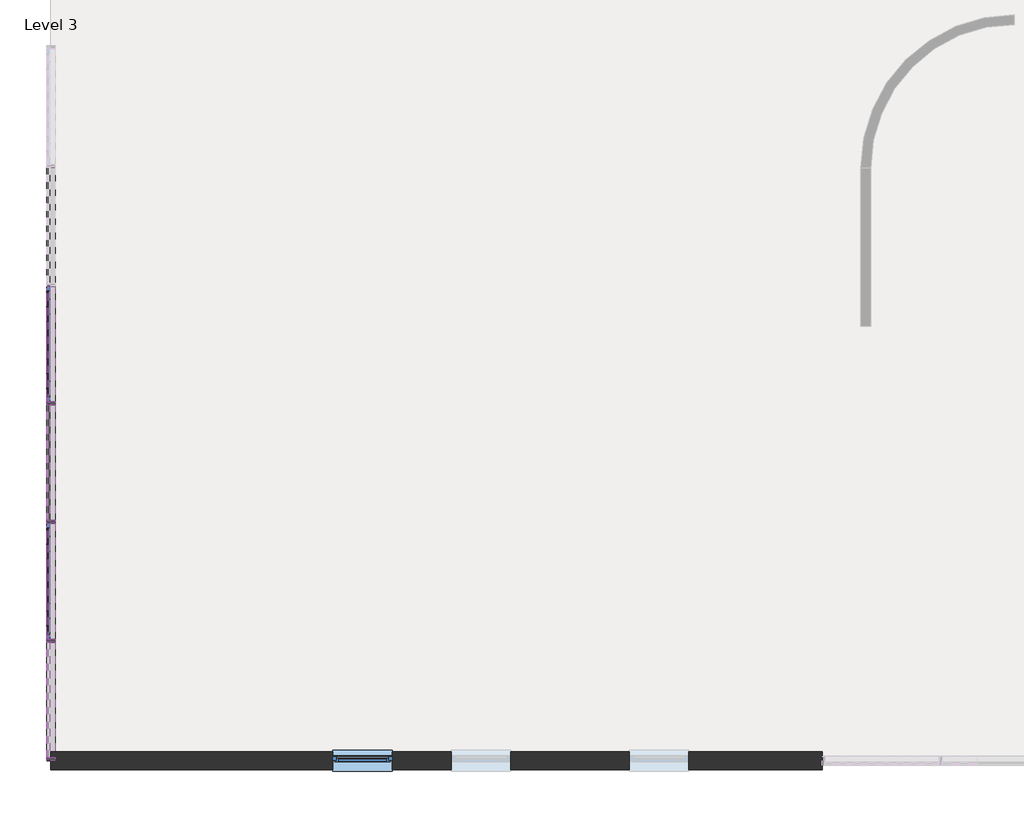
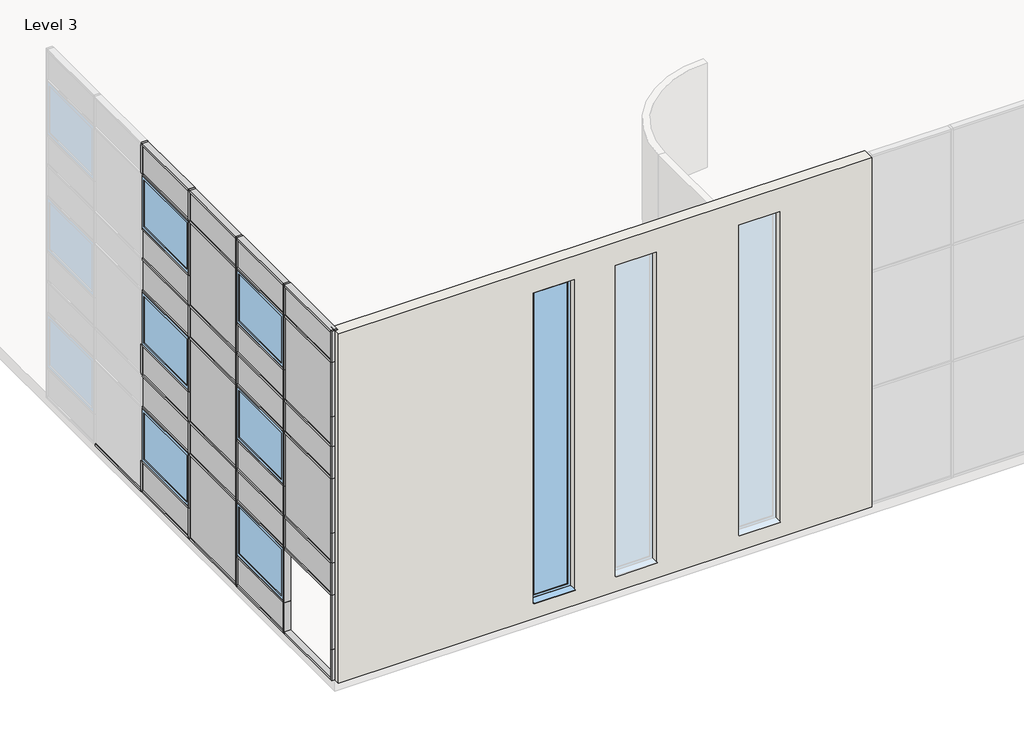
# One storey, part 1 of 5: 74 members, 23 plates, 7 windows, 1 wall.
"""IFC4 building model written with IfcOpenShell, lengths in millimetres."""

import ifcopenshell
import ifcopenshell.guid

model = None  # the IFC model being written
_history = None  # IfcOwnerHistory: only IFC2X3 demands one
_inside = {}  # id of a spatial element -> (the spatial element, [elements in it])
_under = {}  # id of a project, library or spatial element -> (it, [spatial elements below it])
_declared = {}  # id of a project -> (the project, [libraries it declares])
_typed = {}  # id of a type object -> (the type object, [elements of that type])
_made_of = {}  # id of a material, layer set ... -> (it, [elements and type objects made of it])


def new_model(schema):
    """Start an empty IFC model of exactly this schema.

    Asked for "IFC4X3", IfcOpenShell would pick the latest addendum, in which some entities
    have other attributes; the version numbers below select the first issue.
    IFC2X3 requires an IfcOwnerHistory on every rooted entity: one is made here for all.
    """
    global model, _history
    if schema == "IFC4X3":
        model = ifcopenshell.file(schema_version=(4, 3, 0, 0))
    else:
        model = ifcopenshell.file(schema=schema)
    _inside.clear()
    _under.clear()
    _declared.clear()
    _typed.clear()
    _made_of.clear()
    _history = None
    if model.schema == "IFC2X3":
        org = make("IfcOrganization", Name="unknown")
        user = make(
            "IfcPersonAndOrganization",
            ThePerson=make("IfcPerson", FamilyName="unknown"),
            TheOrganization=org,
        )
        app = make(
            "IfcApplication",
            ApplicationDeveloper=org,
            Version="unknown",
            ApplicationFullName="unknown",
            ApplicationIdentifier="unknown",
        )
        _history = make(
            "IfcOwnerHistory",
            OwningUser=user,
            OwningApplication=app,
            ChangeAction="ADDED",
            CreationDate=0,
        )
    return model


def make(cls, **values):
    """One entity of the class cls with the attributes given. An attribute that is None is left unset."""
    return model.create_entity(
        cls, **{name: value for name, value in values.items() if value is not None}
    )


def rooted(cls, **values):
    """An entity with a GlobalId (a new one), such as an element, a storey or a relation."""
    return make(cls, GlobalId=ifcopenshell.guid.new(), OwnerHistory=_history, **values)


def si_unit(unit_type, name, prefix=None):
    """IfcSIUnit, for example si_unit("LENGTHUNIT", "METRE", prefix="MILLI")."""
    return make("IfcSIUnit", UnitType=unit_type, Prefix=prefix, Name=name)


def assignment(units):
    """IfcUnitAssignment: the units of a project."""
    return None if units is None else make("IfcUnitAssignment", Units=units)


def point(xyz):
    """IfcCartesianPoint."""
    return None if xyz is None else make("IfcCartesianPoint", Coordinates=xyz)


def direction(xyz):
    """IfcDirection."""
    return None if xyz is None else make("IfcDirection", DirectionRatios=xyz)


def frame(location, z_axis=None, x_axis=None):
    """IfcAxis2Placement3D, a coordinate frame: its origin and axes. An axis left out is left unset."""
    return make(
        "IfcAxis2Placement3D",
        Location=point(location),
        Axis=direction(z_axis),
        RefDirection=direction(x_axis),
    )


def origin():
    """The frame at (0, 0, 0) with its axes left unset."""
    return frame((0.0, 0.0, 0.0))


def origin_with_axes():
    """The frame at (0, 0, 0) with the z axis (0, 0, 1) and the x axis (1, 0, 0) written out."""
    return frame((0.0, 0.0, 0.0), z_axis=(0.0, 0.0, 1.0), x_axis=(1.0, 0.0, 0.0))


def place(relative_to, where):
    """IfcLocalPlacement: puts the frame where relative to a parent placement (None: the world)."""
    return make(
        "IfcLocalPlacement", PlacementRelTo=relative_to, RelativePlacement=where
    )


def context(
    kind, dimensions, precision=None, world=None, true_north=None, identifier=None
):
    """IfcGeometricRepresentationContext, for example the 3D "Model" context."""
    return make(
        "IfcGeometricRepresentationContext",
        ContextIdentifier=identifier,
        ContextType=kind,
        CoordinateSpaceDimension=dimensions,
        Precision=precision,
        WorldCoordinateSystem=world,
        TrueNorth=true_north,
    )


def project(units=None, contexts=None):
    """IfcProject with its units and contexts."""
    return rooted(
        "IfcProject",
        Name="project",
        RepresentationContexts=contexts,
        UnitsInContext=assignment(units),
    )


def spatial(cls, under=None, at=None, **own):
    """A site, building, storey or space (cls), placed at a placement, below another one or the project."""
    s = rooted(cls, ObjectPlacement=at, **own)
    if under is not None:
        _under.setdefault(under.id(), (under, []))[1].append(s)
    return s


def polyline(points):
    """IfcPolyline through the points."""
    return make("IfcPolyline", Points=[point(p) for p in points])


def outline(outer, holes=None, kind="AREA"):
    """IfcArbitraryClosedProfileDef: a profile drawn as a closed curve; with holes, ...WithVoids."""
    if holes is None:
        return make("IfcArbitraryClosedProfileDef", ProfileType=kind, OuterCurve=outer)
    return make(
        "IfcArbitraryProfileDefWithVoids",
        ProfileType=kind,
        OuterCurve=outer,
        InnerCurves=holes,
    )


def extrude(swept, where, along, depth):
    """IfcExtrudedAreaSolid: the profile swept, set in the frame where, extruded along a direction by depth."""
    return make(
        "IfcExtrudedAreaSolid",
        SweptArea=swept,
        Position=where,
        ExtrudedDirection=direction(along),
        Depth=depth,
    )


def faces_of(points, faces, orient=None, outer=None):
    """IfcFace entities. A face is a list of loops; a loop is a list of indices into points, from 0.

    orient and outer hold one flag for each loop. By default every Orientation is true, the
    first loop of a face is its IfcFaceOuterBound and the others are IfcFaceBound.
    """
    made = []
    for i, loops in enumerate(faces):
        bounds = []
        for j, loop in enumerate(loops):
            is_outer = j == 0 if outer is None else outer[i][j]
            bounds.append(
                make(
                    "IfcFaceOuterBound" if is_outer else "IfcFaceBound",
                    Bound=make("IfcPolyLoop", Polygon=[points[k] for k in loop]),
                    Orientation=True if orient is None else orient[i][j],
                )
            )
        made.append(make("IfcFace", Bounds=bounds))
    return made


def faceted_brep(points, faces, orient=None, outer=None, voids=None):
    """IfcFacetedBrep: a solid bounded by flat faces; with voids (closed shells), ...WithVoids."""
    shared = [point(p) for p in points]
    hull = make("IfcClosedShell", CfsFaces=faces_of(shared, faces, orient, outer))
    if voids is None:
        return make("IfcFacetedBrep", Outer=hull)
    return make(
        "IfcFacetedBrepWithVoids",
        Outer=hull,
        Voids=[
            make(cls, CfsFaces=faces_of(shared, fs, o, b)) for cls, fs, o, b in voids
        ],
    )


def shape(context_of_items, identifier, shape_type, items):
    """IfcShapeRepresentation: the items that make up one representation, for example the "Body"."""
    return make(
        "IfcShapeRepresentation",
        ContextOfItems=context_of_items,
        RepresentationIdentifier=identifier,
        RepresentationType=shape_type,
        Items=items,
    )


def source(mapping_origin, context_of_items, identifier, shape_type, items):
    """IfcRepresentationMap: a shape defined once, which mapped items show again and again."""
    return make(
        "IfcRepresentationMap",
        MappingOrigin=mapping_origin,
        MappedRepresentation=shape(context_of_items, identifier, shape_type, items),
    )


def transform(
    local_origin,
    x_axis=None,
    y_axis=None,
    z_axis=None,
    scale=None,
    scale2=None,
    scale3=None,
    uniform=True,
):
    """IfcCartesianTransformationOperator3D, or its non-uniform kind. x_axis, y_axis, z_axis: its Axis1, 2, 3."""
    if uniform:
        return make(
            "IfcCartesianTransformationOperator3D",
            Axis1=direction(x_axis),
            Axis2=direction(y_axis),
            LocalOrigin=point(local_origin),
            Scale=scale,
            Axis3=direction(z_axis),
        )
    return make(
        "IfcCartesianTransformationOperator3DnonUniform",
        Axis1=direction(x_axis),
        Axis2=direction(y_axis),
        LocalOrigin=point(local_origin),
        Scale=scale,
        Axis3=direction(z_axis),
        Scale2=scale2,
        Scale3=scale3,
    )


def mapped(mapping_source, mapping_target):
    """IfcMappedItem: shows the shape of a source again, moved by a transform."""
    return make(
        "IfcMappedItem", MappingSource=mapping_source, MappingTarget=mapping_target
    )


def made_of(thing, what):
    """Note that an element or type object is made of a material, layer set ...; save() writes the relation."""
    if what is not None:
        _made_of.setdefault(what.id(), (what, []))[1].append(thing)
    return thing


def element(
    cls,
    number,
    at=None,
    inside=None,
    cuts=None,
    type_object=None,
    material=None,
    context=None,
    identifier="Body",
    shape_type=None,
    held_by="IfcProductDefinitionShape",
    body=None,
    shapes=None,
    **own,
):
    """One element of the class cls, such as IfcWall. Its Tag is "e" and its number.

    at: its placement. inside: the storey or other place that contains it. cuts: it is an
    opening in that element (IfcRelVoidsElement). A single representation is given by context,
    identifier, shape_type and body (its items); several are given by shapes. held_by: the class
    of the entity that holds the representations. save() writes the other relations.
    """
    e = rooted(cls, Tag="e%d" % number, ObjectPlacement=at, **own)
    if body is not None:
        shapes = [shape(context, identifier, shape_type, body)]
    if shapes is not None:
        e.Representation = make(held_by, Representations=shapes)
    if inside is not None:
        _inside.setdefault(inside.id(), (inside, []))[1].append(e)
    if cuts is not None:
        rooted(
            "IfcRelVoidsElement", RelatingBuildingElement=cuts, RelatedOpeningElement=e
        )
    if type_object is not None:
        _typed.setdefault(type_object.id(), (type_object, []))[1].append(e)
    return made_of(e, material)


def aggregate(whole, parts):
    """IfcRelAggregates: a whole, such as a stair, and the parts it consists of."""
    return rooted("IfcRelAggregates", RelatingObject=whole, RelatedObjects=parts)


def save(model, path):
    """Write the relations noted so far, then the file.

    IfcRelAggregates (storeys below a building ...), IfcRelContainedInSpatialStructure (elements
    in a storey), IfcRelDefinesByType, IfcRelAssociatesMaterial and IfcRelDeclares: one each for
    every whole, place, type object, material and project.
    """
    for whole, parts in _under.values():
        aggregate(whole, parts)
    for where, things in _inside.values():
        rooted(
            "IfcRelContainedInSpatialStructure",
            RelatedElements=things,
            RelatingStructure=where,
        )
    for kind, things in _typed.values():
        rooted("IfcRelDefinesByType", RelatedObjects=things, RelatingType=kind)
    for what, things in _made_of.values():
        rooted("IfcRelAssociatesMaterial", RelatedObjects=things, RelatingMaterial=what)
    for by, libraries in _declared.values():
        rooted("IfcRelDeclares", RelatingContext=by, RelatedDefinitions=libraries)
    model.write(path)


def rectangular_mullion_50_x_150mm_0967fd3c(model_context):
    return source(origin(), model_context, "Body", "SweptSolid", [
        extrude(outline(polyline([(0.0, 75.0), (0.0, -75.0), (-50.0, -75.0), (-50.0, 75.0), (0.0, 75.0)])), frame((0.0, 0.0, -1950.0000003), z_axis=(0.0, 0.0, 1.0), x_axis=(1.0, 0.0, 0.0)), (0.0, 0.0, 1.0), 1950.0000003),
    ])


def rectangular_mullion_50_x_150mm_f1645b81(model_context):
    return source(origin(), model_context, "Body", "SweptSolid", [
        extrude(outline(polyline([(25.0, 75.0), (25.0, -75.0), (-25.0, -75.0), (-25.0, 75.0), (25.0, 75.0)])), frame((0.0, 0.0, -1950.0000003), z_axis=(0.0, 0.0, 1.0), x_axis=(1.0, 0.0, 0.0)), (0.0, 0.0, 1.0), 1950.0000003),
    ])


def rectangular_mullion_50_x_150mm_14f10ac7(model_context):
    return source(origin(), model_context, "Body", "SweptSolid", [
        extrude(outline(polyline([(25.0, 75.0), (25.0, -75.0), (-25.0, -75.0), (-25.0, 75.0), (25.0, 75.0)])), frame((0.0, 0.0, -800.0), z_axis=(0.0, 0.0, 1.0), x_axis=(1.0, 0.0, 0.0)), (0.0, 0.0, 1.0), 800.0),
    ])


def rectangular_mullion_50_x_150mm_6270d9f9(model_context):
    return source(origin(), model_context, "Body", "SweptSolid", [
        extrude(outline(polyline([(25.0, 75.0), (25.0, -75.0), (-25.0, -75.0), (-25.0, 75.0), (25.0, 75.0)])), frame((0.0, 0.0, -775.0), z_axis=(0.0, 0.0, 1.0), x_axis=(1.0, 0.0, 0.0)), (0.0, 0.0, 1.0), 775.0),
    ])


def rectangular_mullion_50_x_150mm_80d7b263(model_context):
    return source(origin(), model_context, "Body", "SweptSolid", [
        extrude(outline(polyline([(25.0, 75.0), (25.0, -75.0), (-25.0, -75.0), (-25.0, 75.0), (25.0, 75.0)])), frame((0.0, 0.0, -1400.0), z_axis=(0.0, 0.0, 1.0), x_axis=(1.0, 0.0, 0.0)), (0.0, 0.0, 1.0), 1400.0),
    ])


def rectangular_mullion_50_x_150mm_9c26cac3(model_context):
    return source(origin(), model_context, "Body", "SweptSolid", [
        extrude(outline(polyline([(25.0, 75.0), (25.0, -75.0), (-25.0, -75.0), (-25.0, 75.0), (25.0, 75.0)])), frame((0.0, 0.0, -825.0), z_axis=(0.0, 0.0, 1.0), x_axis=(1.0, 0.0, 0.0)), (0.0, 0.0, 1.0), 825.0),
    ])


def rectangular_mullion_50_x_150mm_6ffebc0f(model_context):
    return source(origin(), model_context, "Body", "SweptSolid", [
        extrude(outline(polyline([(0.0, 75.0), (0.0, -75.0), (-50.0, -75.0), (-50.0, 75.0), (0.0, 75.0)])), frame((0.0, 0.0, -800.0), z_axis=(0.0, 0.0, 1.0), x_axis=(1.0, 0.0, 0.0)), (0.0, 0.0, 1.0), 800.0),
    ])


def rectangular_mullion_50_x_150mm_0ac3c94c(model_context):
    return source(origin(), model_context, "Body", "SweptSolid", [
        extrude(outline(polyline([(0.0, 75.0), (0.0, -75.0), (-50.0, -75.0), (-50.0, 75.0), (0.0, 75.0)])), frame((0.0, 0.0, -1400.0), z_axis=(0.0, 0.0, 1.0), x_axis=(1.0, 0.0, 0.0)), (0.0, 0.0, 1.0), 1400.0),
    ])


def rectangular_mullion_50_x_150mm_4883e7f1(model_context):
    return source(origin(), model_context, "Body", "SweptSolid", [
        extrude(outline(polyline([(0.0, 75.0), (0.0, -75.0), (-50.0, -75.0), (-50.0, 75.0), (0.0, 75.0)])), frame((0.0, 0.0, -825.0), z_axis=(0.0, 0.0, 1.0), x_axis=(1.0, 0.0, 0.0)), (0.0, 0.0, 1.0), 825.0),
    ])


def rectangular_mullion_50_x_150mm_5dc04e1f(model_context):
    return source(origin(), model_context, "Body", "SweptSolid", [
        extrude(outline(polyline([(0.0, 75.0), (0.0, -75.0), (-50.0, -75.0), (-50.0, 75.0), (0.0, 75.0)])), frame((0.0, 0.0, -775.0), z_axis=(0.0, 0.0, 1.0), x_axis=(1.0, 0.0, 0.0)), (0.0, 0.0, 1.0), 775.0),
    ])


def system_panel_glazed_1e38db9b(model_context):
    return source(origin(), model_context, "Body", "SweptSolid", [
        extrude(outline(polyline([(0.0, -975.0000002), (0.0, 975.0000002), (750.0, 975.0000002), (2125.0, 975.0000002), (2125.0, -975.0000002), (750.0, -975.0000002), (0.0, -975.0000002)])), frame((0.0, 24.5, 0.0), z_axis=(0.0, 1.0, 0.0), x_axis=(0.0, 0.0, 1.0)), (0.0, 0.0, 1.0), 25.0),
    ])


def system_panel_glazed_bc1ebc0c(model_context):
    return source(origin(), model_context, "Body", "SweptSolid", [
        extrude(outline(polyline([(975.0000002, 24.5), (-975.0000002, 24.5), (-975.0000002, 49.5), (975.0000002, 49.5), (975.0000002, 24.5)])), origin_with_axes(), (0.0, 0.0, 1.0), 725.0),
    ])


def system_panel_glazed_d82c9dbb(model_context):
    return source(origin(), model_context, "Body", "SweptSolid", [
        extrude(outline(polyline([(975.0000002, 24.5), (-975.0000002, 24.5), (-975.0000002, 49.5), (975.0000002, 49.5), (975.0000002, 24.5)])), origin_with_axes(), (0.0, 0.0, 1.0), 775.0),
    ])


def m_curtain_wall_awning_m_curtain_wall_awning_db665c81(model_context):
    return source(origin(), model_context, "Body", "SweptSolid", [
        extrude(outline(polyline([(900.0, 44.05), (-900.0, 44.05), (-900.0, 56.75), (900.0, 56.75), (900.0, 44.05)])), frame((0.0, 0.0, 75.0), z_axis=(0.0, 0.0, 1.0), x_axis=(1.0, 0.0, 0.0)), (0.0, 0.0, 1.0), 1200.0),
        extrude(outline(polyline([(1350.0, -975.0), (0.0, -975.0), (0.0, 975.0), (1350.0, 975.0), (1350.0, -975.0)]), holes=[polyline([(1275.0, -900.0), (1275.0, 900.0), (75.0, 900.0), (75.0, -900.0), (1275.0, -900.0)])]), frame((0.0, 25.0, 0.0), z_axis=(0.0, 1.0, 0.0), x_axis=(0.0, 0.0, 1.0)), (0.0, 0.0, 1.0), 50.0),
    ])


def window_variable_standard_9eb8f332(model_context):
    return source(origin(), model_context, "Body", "SolidModel", [
        extrude(outline(polyline([(9000.0, 500.0), (9000.0, -500.0), (1000.0, -500.0), (1000.0, 500.0), (9000.0, 500.0)]), holes=[polyline([(8920.0, 440.0), (1080.0, 440.0), (1080.0, -440.0), (8920.0, -440.0), (8920.0, 440.0)])]), frame((0.0, -70.0, 0.0), z_axis=(0.0, 1.0, 0.0), x_axis=(0.0, 0.0, 1.0)), (0.0, 0.0, 1.0), 60.0),
        faceted_brep([(470.0, -10.0, 8950.0), (470.0, -10.0, 1050.0), (470.0, 20.0, 1050.0), (470.0, 20.0, 8950.0), (-470.0, 20.0, 1050.0), (-470.0, 20.0, 8950.0), (410.0, 20.0, 1110.0), (410.0, 20.0, 8890.0), (-410.0, 20.0, 8890.0), (-410.0, 20.0, 1110.0), (-470.0, -10.0, 1050.0), (-470.0, -10.0, 8950.0), (440.0, -10.0, 8920.0), (440.0, -10.0, 1080.0), (-440.0, -10.0, 1080.0), (-440.0, -10.0, 8920.0), (440.0, -40.0, 8920.0), (440.0, -40.0, 1080.0), (-440.0, -40.0, 1080.0), (-440.0, -40.0, 8920.0), (410.0, -40.0, 8890.0), (410.0, -40.0, 1110.0), (-410.0, -40.0, 1110.0), (-410.0, -40.0, 8890.0)], [[[0, 1, 2, 3]], [[3, 2, 4, 5], [6, 7, 8, 9]], [[1, 10, 4, 2]], [[1, 0, 11, 10], [12, 13, 14, 15]], [[16, 17, 13, 12]], [[17, 18, 14, 13]], [[17, 16, 19, 18], [20, 21, 22, 23]], [[7, 6, 21, 20]], [[6, 9, 22, 21]], [[10, 11, 5, 4]], [[18, 19, 15, 14]], [[9, 8, 23, 22]], [[11, 0, 3, 5]], [[19, 16, 12, 15]], [[8, 7, 20, 23]]]),
        extrude(outline(polyline([(-500.0, 180.0), (500.0, 180.0), (500.0, -10.0), (-500.0, -10.0), (-500.0, 180.0)])), frame((0.0, 0.0, 1005.0), z_axis=(0.0, 0.0, 1.0), x_axis=(1.0, 0.0, 0.0)), (0.0, 0.0, 1.0), 15.0),
        extrude(outline(polyline([(-80.0221543, 1020.0), (-70.0, 1020.0), (-70.0, 1018.0), (-79.8240723, 1018.0), (-178.0, 998.3604634), (-178.0, 990.0), (-180.0, 990.0), (-180.0, 1000.0), (-80.0221543, 1020.0)])), frame((-500.0, 0.0, 0.0), z_axis=(1.0, 0.0, 0.0), x_axis=(0.0, 1.0, 0.0)), (0.0, 0.0, 1.0), 1000.0),
        extrude(outline(polyline([(410.0, 5.0), (410.0, -25.0), (-410.0, -25.0), (-410.0, 5.0), (410.0, 5.0)])), frame((0.0, 0.0, 1110.0), z_axis=(0.0, 0.0, 1.0), x_axis=(1.0, 0.0, 0.0)), (0.0, 0.0, 1.0), 7780.0),
    ])


model = new_model("IFC4")

# Units and contexts
model_context = context("Model", 3, world=origin())
ifc_project = project(units=[si_unit("LENGTHUNIT", "METRE", prefix="MILLI")], contexts=[model_context])

# Site, building, storey
site = spatial("IfcSite", under=ifc_project)
building = spatial("IfcBuilding", under=site)
storey = spatial("IfcBuildingStorey", under=building, Name="Level 3", Elevation=6000.0)

# Members
placement = place(None, origin())
rectangular_mullion_50_x_150mm_shape = rectangular_mullion_50_x_150mm_0967fd3c(model_context)
element("IfcMember", 1, ObjectType="Rectangular Mullion : 50 x 150mm", at=placement, inside=storey, context=model_context, shape_type="MappedRepresentation", body=[
    mapped(rectangular_mullion_50_x_150mm_shape, transform((-6732.0028633, -9951.242277, 6000.0), x_axis=(0.0, 0.0, -1.0), y_axis=(1.0, 0.0, 0.0), z_axis=(0.0, -1.0, 0.0))),
])
element("IfcMember", 2, ObjectType="Rectangular Mullion : 50 x 150mm", at=placement, inside=storey, context=model_context, shape_type="MappedRepresentation", body=[
    mapped(rectangular_mullion_50_x_150mm_shape, transform((-6732.0028633, -7951.2422767, 6000.0), x_axis=(0.0, 0.0, -1.0), y_axis=(1.0, 0.0, 0.0), z_axis=(0.0, -1.0, 0.0))),
])
element("IfcMember", 3, ObjectType="Rectangular Mullion : 50 x 150mm", at=placement, inside=storey, context=model_context, shape_type="MappedRepresentation", body=[
    mapped(rectangular_mullion_50_x_150mm_shape, transform((-6732.0028633, -5951.2422767, 6000.0), x_axis=(0.0, 0.0, -1.0), y_axis=(1.0, 0.0, 0.0), z_axis=(0.0, -1.0, 0.0))),
])
element("IfcMember", 4, ObjectType="Rectangular Mullion : 50 x 150mm", at=placement, inside=storey, context=model_context, shape_type="MappedRepresentation", body=[
    mapped(rectangular_mullion_50_x_150mm_shape, transform((-6732.0028633, -3951.2422767, 6000.0), x_axis=(0.0, 0.0, -1.0), y_axis=(1.0, 0.0, 0.0), z_axis=(0.0, -1.0, 0.0))),
])
element("IfcMember", 5, ObjectType="Rectangular Mullion : 50 x 150mm", at=placement, inside=storey, context=model_context, shape_type="MappedRepresentation", body=[
    mapped(rectangular_mullion_50_x_150mm_shape, transform((-6732.0028633, -1951.2422767, 6000.0), x_axis=(0.0, 0.0, -1.0), y_axis=(1.0, 0.0, 0.0), z_axis=(0.0, -1.0, 0.0))),
])
rectangular_mullion_50_x_150mm_2_shape = rectangular_mullion_50_x_150mm_f1645b81(model_context)
element("IfcMember", 6, ObjectType="Rectangular Mullion : 50 x 150mm", at=placement, inside=storey, context=model_context, shape_type="MappedRepresentation", body=[
    mapped(rectangular_mullion_50_x_150mm_2_shape, transform((-6732.0028633, -8001.2422767, 14200.0), x_axis=(0.0, 0.0, 1.0), y_axis=(1.0, 0.0, 0.0), z_axis=(0.0, 1.0, 0.0))),
])
element("IfcMember", 7, ObjectType="Rectangular Mullion : 50 x 150mm", at=placement, inside=storey, context=model_context, shape_type="MappedRepresentation", body=[
    mapped(rectangular_mullion_50_x_150mm_2_shape, transform((-6732.0028633, -6001.2422767, 14200.0), x_axis=(0.0, 0.0, 1.0), y_axis=(1.0, 0.0, 0.0), z_axis=(0.0, 1.0, 0.0))),
])
element("IfcMember", 8, ObjectType="Rectangular Mullion : 50 x 150mm", at=placement, inside=storey, context=model_context, shape_type="MappedRepresentation", body=[
    mapped(rectangular_mullion_50_x_150mm_2_shape, transform((-6732.0028633, -4001.2422767, 14200.0), x_axis=(0.0, 0.0, 1.0), y_axis=(1.0, 0.0, 0.0), z_axis=(0.0, 1.0, 0.0))),
])
element("IfcMember", 9, ObjectType="Rectangular Mullion : 50 x 150mm", at=placement, inside=storey, context=model_context, shape_type="MappedRepresentation", body=[
    mapped(rectangular_mullion_50_x_150mm_2_shape, transform((-6732.0028633, -2001.2422767, 14200.0), x_axis=(0.0, 0.0, 1.0), y_axis=(1.0, 0.0, 0.0), z_axis=(0.0, 1.0, 0.0))),
])
element("IfcMember", 10, ObjectType="Rectangular Mullion : 50 x 150mm", at=placement, inside=storey, context=model_context, shape_type="MappedRepresentation", body=[
    mapped(rectangular_mullion_50_x_150mm_2_shape, transform((-6732.0028633, -8001.2422767, 9025.0), x_axis=(0.0, 0.0, 1.0), y_axis=(1.0, 0.0, 0.0), z_axis=(0.0, 1.0, 0.0))),
])
element("IfcMember", 11, ObjectType="Rectangular Mullion : 50 x 150mm", at=placement, inside=storey, context=model_context, shape_type="MappedRepresentation", body=[
    mapped(rectangular_mullion_50_x_150mm_2_shape, transform((-6732.0028633, -6001.2422767, 9025.0), x_axis=(0.0, 0.0, 1.0), y_axis=(1.0, 0.0, 0.0), z_axis=(0.0, 1.0, 0.0))),
])
element("IfcMember", 12, ObjectType="Rectangular Mullion : 50 x 150mm", at=placement, inside=storey, context=model_context, shape_type="MappedRepresentation", body=[
    mapped(rectangular_mullion_50_x_150mm_2_shape, transform((-6732.0028633, -4001.2422767, 9025.0), x_axis=(0.0, 0.0, 1.0), y_axis=(1.0, 0.0, 0.0), z_axis=(0.0, 1.0, 0.0))),
])
element("IfcMember", 13, ObjectType="Rectangular Mullion : 50 x 150mm", at=placement, inside=storey, context=model_context, shape_type="MappedRepresentation", body=[
    mapped(rectangular_mullion_50_x_150mm_2_shape, transform((-6732.0028633, -2001.2422767, 9025.0), x_axis=(0.0, 0.0, 1.0), y_axis=(1.0, 0.0, 0.0), z_axis=(0.0, 1.0, 0.0))),
])
element("IfcMember", 14, ObjectType="Rectangular Mullion : 50 x 150mm", at=placement, inside=storey, context=model_context, shape_type="MappedRepresentation", body=[
    mapped(rectangular_mullion_50_x_150mm_2_shape, transform((-6732.0028633, -8001.2422767, 12025.0), x_axis=(0.0, 0.0, 1.0), y_axis=(1.0, 0.0, 0.0), z_axis=(0.0, 1.0, 0.0))),
])
element("IfcMember", 15, ObjectType="Rectangular Mullion : 50 x 150mm", at=placement, inside=storey, context=model_context, shape_type="MappedRepresentation", body=[
    mapped(rectangular_mullion_50_x_150mm_2_shape, transform((-6732.0028633, -6001.2422767, 12025.0), x_axis=(0.0, 0.0, 1.0), y_axis=(1.0, 0.0, 0.0), z_axis=(0.0, 1.0, 0.0))),
])
element("IfcMember", 16, ObjectType="Rectangular Mullion : 50 x 150mm", at=placement, inside=storey, context=model_context, shape_type="MappedRepresentation", body=[
    mapped(rectangular_mullion_50_x_150mm_2_shape, transform((-6732.0028633, -4001.2422767, 12025.0), x_axis=(0.0, 0.0, 1.0), y_axis=(1.0, 0.0, 0.0), z_axis=(0.0, 1.0, 0.0))),
])
element("IfcMember", 17, ObjectType="Rectangular Mullion : 50 x 150mm", at=placement, inside=storey, context=model_context, shape_type="MappedRepresentation", body=[
    mapped(rectangular_mullion_50_x_150mm_2_shape, transform((-6732.0028633, -2001.2422767, 12025.0), x_axis=(0.0, 0.0, 1.0), y_axis=(1.0, 0.0, 0.0), z_axis=(0.0, 1.0, 0.0))),
])
element("IfcMember", 18, ObjectType="Rectangular Mullion : 50 x 150mm", at=placement, inside=storey, context=model_context, shape_type="MappedRepresentation", body=[
    mapped(rectangular_mullion_50_x_150mm_2_shape, transform((-6732.0028633, -6001.2422767, 12800.0), x_axis=(0.0, 0.0, 1.0), y_axis=(1.0, 0.0, 0.0), z_axis=(0.0, 1.0, 0.0))),
])
element("IfcMember", 19, ObjectType="Rectangular Mullion : 50 x 150mm", at=placement, inside=storey, context=model_context, shape_type="MappedRepresentation", body=[
    mapped(rectangular_mullion_50_x_150mm_2_shape, transform((-6732.0028633, -2001.2422767, 12800.0), x_axis=(0.0, 0.0, 1.0), y_axis=(1.0, 0.0, 0.0), z_axis=(0.0, 1.0, 0.0))),
])
element("IfcMember", 20, ObjectType="Rectangular Mullion : 50 x 150mm", at=placement, inside=storey, context=model_context, shape_type="MappedRepresentation", body=[
    mapped(rectangular_mullion_50_x_150mm_2_shape, transform((-6732.0028633, -8001.2422767, 11200.0), x_axis=(0.0, 0.0, 1.0), y_axis=(1.0, 0.0, 0.0), z_axis=(0.0, 1.0, 0.0))),
])
element("IfcMember", 21, ObjectType="Rectangular Mullion : 50 x 150mm", at=placement, inside=storey, context=model_context, shape_type="MappedRepresentation", body=[
    mapped(rectangular_mullion_50_x_150mm_2_shape, transform((-6732.0028633, -6001.2422767, 11200.0), x_axis=(0.0, 0.0, 1.0), y_axis=(1.0, 0.0, 0.0), z_axis=(0.0, 1.0, 0.0))),
])
element("IfcMember", 22, ObjectType="Rectangular Mullion : 50 x 150mm", at=placement, inside=storey, context=model_context, shape_type="MappedRepresentation", body=[
    mapped(rectangular_mullion_50_x_150mm_2_shape, transform((-6732.0028633, -4001.2422767, 11200.0), x_axis=(0.0, 0.0, 1.0), y_axis=(1.0, 0.0, 0.0), z_axis=(0.0, 1.0, 0.0))),
])
element("IfcMember", 23, ObjectType="Rectangular Mullion : 50 x 150mm", at=placement, inside=storey, context=model_context, shape_type="MappedRepresentation", body=[
    mapped(rectangular_mullion_50_x_150mm_2_shape, transform((-6732.0028633, -2001.2422767, 11200.0), x_axis=(0.0, 0.0, 1.0), y_axis=(1.0, 0.0, 0.0), z_axis=(0.0, 1.0, 0.0))),
])
element("IfcMember", 24, ObjectType="Rectangular Mullion : 50 x 150mm", at=placement, inside=storey, context=model_context, shape_type="MappedRepresentation", body=[
    mapped(rectangular_mullion_50_x_150mm_2_shape, transform((-6732.0028633, -6001.2422767, 9800.0), x_axis=(0.0, 0.0, 1.0), y_axis=(1.0, 0.0, 0.0), z_axis=(0.0, 1.0, 0.0))),
])
element("IfcMember", 25, ObjectType="Rectangular Mullion : 50 x 150mm", at=placement, inside=storey, context=model_context, shape_type="MappedRepresentation", body=[
    mapped(rectangular_mullion_50_x_150mm_2_shape, transform((-6732.0028633, -2001.2422767, 9800.0), x_axis=(0.0, 0.0, 1.0), y_axis=(1.0, 0.0, 0.0), z_axis=(0.0, 1.0, 0.0))),
])
element("IfcMember", 26, ObjectType="Rectangular Mullion : 50 x 150mm", at=placement, inside=storey, context=model_context, shape_type="MappedRepresentation", body=[
    mapped(rectangular_mullion_50_x_150mm_2_shape, transform((-6732.0028633, -8001.2422767, 8200.0), x_axis=(0.0, 0.0, 1.0), y_axis=(1.0, 0.0, 0.0), z_axis=(0.0, 1.0, 0.0))),
])
element("IfcMember", 27, ObjectType="Rectangular Mullion : 50 x 150mm", at=placement, inside=storey, context=model_context, shape_type="MappedRepresentation", body=[
    mapped(rectangular_mullion_50_x_150mm_2_shape, transform((-6732.0028633, -6001.2422767, 8200.0), x_axis=(0.0, 0.0, 1.0), y_axis=(1.0, 0.0, 0.0), z_axis=(0.0, 1.0, 0.0))),
])
element("IfcMember", 28, ObjectType="Rectangular Mullion : 50 x 150mm", at=placement, inside=storey, context=model_context, shape_type="MappedRepresentation", body=[
    mapped(rectangular_mullion_50_x_150mm_2_shape, transform((-6732.0028633, -4001.2422767, 8200.0), x_axis=(0.0, 0.0, 1.0), y_axis=(1.0, 0.0, 0.0), z_axis=(0.0, 1.0, 0.0))),
])
element("IfcMember", 29, ObjectType="Rectangular Mullion : 50 x 150mm", at=placement, inside=storey, context=model_context, shape_type="MappedRepresentation", body=[
    mapped(rectangular_mullion_50_x_150mm_2_shape, transform((-6732.0028633, -2001.2422767, 8200.0), x_axis=(0.0, 0.0, 1.0), y_axis=(1.0, 0.0, 0.0), z_axis=(0.0, 1.0, 0.0))),
])
element("IfcMember", 30, ObjectType="Rectangular Mullion : 50 x 150mm", at=placement, inside=storey, context=model_context, shape_type="MappedRepresentation", body=[
    mapped(rectangular_mullion_50_x_150mm_2_shape, transform((-6732.0028633, -6001.2422767, 6800.0), x_axis=(0.0, 0.0, 1.0), y_axis=(1.0, 0.0, 0.0), z_axis=(0.0, 1.0, 0.0))),
])
element("IfcMember", 31, ObjectType="Rectangular Mullion : 50 x 150mm", at=placement, inside=storey, context=model_context, shape_type="MappedRepresentation", body=[
    mapped(rectangular_mullion_50_x_150mm_2_shape, transform((-6732.0028633, -2001.2422767, 6800.0), x_axis=(0.0, 0.0, 1.0), y_axis=(1.0, 0.0, 0.0), z_axis=(0.0, 1.0, 0.0))),
])
rectangular_mullion_50_x_150mm_3_shape = rectangular_mullion_50_x_150mm_14f10ac7(model_context)
element("IfcMember", 32, ObjectType="Rectangular Mullion : 50 x 150mm", at=placement, inside=storey, context=model_context, shape_type="MappedRepresentation", body=[
    mapped(rectangular_mullion_50_x_150mm_3_shape, transform((-6732.0028633, -7976.2422767, 6000.0), x_axis=(0.0, 1.0, 0.0), y_axis=(1.0, 0.0, 0.0), z_axis=(0.0, 0.0, -1.0))),
])
element("IfcMember", 33, ObjectType="Rectangular Mullion : 50 x 150mm", at=placement, inside=storey, context=model_context, shape_type="MappedRepresentation", body=[
    mapped(rectangular_mullion_50_x_150mm_3_shape, transform((-6732.0028633, -5976.2422767, 6000.0), x_axis=(0.0, 1.0, 0.0), y_axis=(1.0, 0.0, 0.0), z_axis=(0.0, 0.0, -1.0))),
])
element("IfcMember", 34, ObjectType="Rectangular Mullion : 50 x 150mm", at=placement, inside=storey, context=model_context, shape_type="MappedRepresentation", body=[
    mapped(rectangular_mullion_50_x_150mm_3_shape, transform((-6732.0028633, -3976.2422767, 6000.0), x_axis=(0.0, 1.0, 0.0), y_axis=(1.0, 0.0, 0.0), z_axis=(0.0, 0.0, -1.0))),
])
element("IfcMember", 35, ObjectType="Rectangular Mullion : 50 x 150mm", at=placement, inside=storey, context=model_context, shape_type="MappedRepresentation", body=[
    mapped(rectangular_mullion_50_x_150mm_3_shape, transform((-6732.0028633, -1976.2422767, 6000.0), x_axis=(0.0, 1.0, 0.0), y_axis=(1.0, 0.0, 0.0), z_axis=(0.0, 0.0, -1.0))),
])
element("IfcMember", 36, ObjectType="Rectangular Mullion : 50 x 150mm", at=placement, inside=storey, context=model_context, shape_type="MappedRepresentation", body=[
    mapped(rectangular_mullion_50_x_150mm_shape, transform((-6732.0028633, -8001.2422767, 15000.0), x_axis=(0.0, 0.0, 1.0), y_axis=(1.0, 0.0, 0.0), z_axis=(0.0, 1.0, 0.0))),
])
element("IfcMember", 37, ObjectType="Rectangular Mullion : 50 x 150mm", at=placement, inside=storey, context=model_context, shape_type="MappedRepresentation", body=[
    mapped(rectangular_mullion_50_x_150mm_shape, transform((-6732.0028633, -6001.2422767, 15000.0), x_axis=(0.0, 0.0, 1.0), y_axis=(1.0, 0.0, 0.0), z_axis=(0.0, 1.0, 0.0))),
])
element("IfcMember", 38, ObjectType="Rectangular Mullion : 50 x 150mm", at=placement, inside=storey, context=model_context, shape_type="MappedRepresentation", body=[
    mapped(rectangular_mullion_50_x_150mm_shape, transform((-6732.0028633, -4001.2422767, 15000.0), x_axis=(0.0, 0.0, 1.0), y_axis=(1.0, 0.0, 0.0), z_axis=(0.0, 1.0, 0.0))),
])
element("IfcMember", 39, ObjectType="Rectangular Mullion : 50 x 150mm", at=placement, inside=storey, context=model_context, shape_type="MappedRepresentation", body=[
    mapped(rectangular_mullion_50_x_150mm_shape, transform((-6732.0028633, -2001.2422767, 15000.0), x_axis=(0.0, 0.0, 1.0), y_axis=(1.0, 0.0, 0.0), z_axis=(0.0, 1.0, 0.0))),
])
element("IfcMember", 40, ObjectType="Rectangular Mullion : 50 x 150mm", at=placement, inside=storey, context=model_context, shape_type="MappedRepresentation", body=[
    mapped(rectangular_mullion_50_x_150mm_3_shape, transform((-6732.0028633, -7976.2422767, 14200.0), x_axis=(0.0, 1.0, 0.0), y_axis=(1.0, 0.0, 0.0), z_axis=(0.0, 0.0, -1.0))),
])
element("IfcMember", 41, ObjectType="Rectangular Mullion : 50 x 150mm", at=placement, inside=storey, context=model_context, shape_type="MappedRepresentation", body=[
    mapped(rectangular_mullion_50_x_150mm_3_shape, transform((-6732.0028633, -5976.2422767, 14200.0), x_axis=(0.0, 1.0, 0.0), y_axis=(1.0, 0.0, 0.0), z_axis=(0.0, 0.0, -1.0))),
])
element("IfcMember", 42, ObjectType="Rectangular Mullion : 50 x 150mm", at=placement, inside=storey, context=model_context, shape_type="MappedRepresentation", body=[
    mapped(rectangular_mullion_50_x_150mm_3_shape, transform((-6732.0028633, -3976.2422767, 14200.0), x_axis=(0.0, 1.0, 0.0), y_axis=(1.0, 0.0, 0.0), z_axis=(0.0, 0.0, -1.0))),
])
element("IfcMember", 43, ObjectType="Rectangular Mullion : 50 x 150mm", at=placement, inside=storey, context=model_context, shape_type="MappedRepresentation", body=[
    mapped(rectangular_mullion_50_x_150mm_3_shape, transform((-6732.0028633, -1976.2422767, 14200.0), x_axis=(0.0, 1.0, 0.0), y_axis=(1.0, 0.0, 0.0), z_axis=(0.0, 0.0, -1.0))),
])
rectangular_mullion_50_x_150mm_4_shape = rectangular_mullion_50_x_150mm_6270d9f9(model_context)
element("IfcMember", 44, ObjectType="Rectangular Mullion : 50 x 150mm", at=placement, inside=storey, context=model_context, shape_type="MappedRepresentation", body=[
    mapped(rectangular_mullion_50_x_150mm_4_shape, transform((-6732.0028633, -7976.2422767, 9025.0), x_axis=(0.0, 1.0, 0.0), y_axis=(1.0, 0.0, 0.0), z_axis=(0.0, 0.0, -1.0))),
])
element("IfcMember", 45, ObjectType="Rectangular Mullion : 50 x 150mm", at=placement, inside=storey, context=model_context, shape_type="MappedRepresentation", body=[
    mapped(rectangular_mullion_50_x_150mm_4_shape, transform((-6732.0028633, -7976.2422767, 12025.0), x_axis=(0.0, 1.0, 0.0), y_axis=(1.0, 0.0, 0.0), z_axis=(0.0, 0.0, -1.0))),
])
element("IfcMember", 46, ObjectType="Rectangular Mullion : 50 x 150mm", at=placement, inside=storey, context=model_context, shape_type="MappedRepresentation", body=[
    mapped(rectangular_mullion_50_x_150mm_4_shape, transform((-6732.0028633, -5976.2422767, 9025.0), x_axis=(0.0, 1.0, 0.0), y_axis=(1.0, 0.0, 0.0), z_axis=(0.0, 0.0, -1.0))),
])
element("IfcMember", 47, ObjectType="Rectangular Mullion : 50 x 150mm", at=placement, inside=storey, context=model_context, shape_type="MappedRepresentation", body=[
    mapped(rectangular_mullion_50_x_150mm_4_shape, transform((-6732.0028633, -5976.2422767, 12025.0), x_axis=(0.0, 1.0, 0.0), y_axis=(1.0, 0.0, 0.0), z_axis=(0.0, 0.0, -1.0))),
])
element("IfcMember", 48, ObjectType="Rectangular Mullion : 50 x 150mm", at=placement, inside=storey, context=model_context, shape_type="MappedRepresentation", body=[
    mapped(rectangular_mullion_50_x_150mm_4_shape, transform((-6732.0028633, -3976.2422767, 9025.0), x_axis=(0.0, 1.0, 0.0), y_axis=(1.0, 0.0, 0.0), z_axis=(0.0, 0.0, -1.0))),
])
element("IfcMember", 49, ObjectType="Rectangular Mullion : 50 x 150mm", at=placement, inside=storey, context=model_context, shape_type="MappedRepresentation", body=[
    mapped(rectangular_mullion_50_x_150mm_4_shape, transform((-6732.0028633, -3976.2422767, 12025.0), x_axis=(0.0, 1.0, 0.0), y_axis=(1.0, 0.0, 0.0), z_axis=(0.0, 0.0, -1.0))),
])
element("IfcMember", 50, ObjectType="Rectangular Mullion : 50 x 150mm", at=placement, inside=storey, context=model_context, shape_type="MappedRepresentation", body=[
    mapped(rectangular_mullion_50_x_150mm_4_shape, transform((-6732.0028633, -1976.2422767, 9025.0), x_axis=(0.0, 1.0, 0.0), y_axis=(1.0, 0.0, 0.0), z_axis=(0.0, 0.0, -1.0))),
])
rectangular_mullion_50_x_150mm_5_shape = rectangular_mullion_50_x_150mm_80d7b263(model_context)
element("IfcMember", 51, ObjectType="Rectangular Mullion : 50 x 150mm", at=placement, inside=storey, context=model_context, shape_type="MappedRepresentation", body=[
    mapped(rectangular_mullion_50_x_150mm_5_shape, transform((-6732.0028633, -7976.2422767, 12800.0), x_axis=(0.0, 1.0, 0.0), y_axis=(1.0, 0.0, 0.0), z_axis=(0.0, 0.0, -1.0))),
])
element("IfcMember", 52, ObjectType="Rectangular Mullion : 50 x 150mm", at=placement, inside=storey, context=model_context, shape_type="MappedRepresentation", body=[
    mapped(rectangular_mullion_50_x_150mm_5_shape, transform((-6732.0028633, -7976.2422767, 9800.0), x_axis=(0.0, 1.0, 0.0), y_axis=(1.0, 0.0, 0.0), z_axis=(0.0, 0.0, -1.0))),
])
element("IfcMember", 53, ObjectType="Rectangular Mullion : 50 x 150mm", at=placement, inside=storey, context=model_context, shape_type="MappedRepresentation", body=[
    mapped(rectangular_mullion_50_x_150mm_5_shape, transform((-6732.0028633, -7976.2422767, 6800.0), x_axis=(0.0, 1.0, 0.0), y_axis=(1.0, 0.0, 0.0), z_axis=(0.0, 0.0, -1.0))),
])
element("IfcMember", 54, ObjectType="Rectangular Mullion : 50 x 150mm", at=placement, inside=storey, context=model_context, shape_type="MappedRepresentation", body=[
    mapped(rectangular_mullion_50_x_150mm_5_shape, transform((-6732.0028633, -5976.2422767, 12800.0), x_axis=(0.0, 1.0, 0.0), y_axis=(1.0, 0.0, 0.0), z_axis=(0.0, 0.0, -1.0))),
])
element("IfcMember", 55, ObjectType="Rectangular Mullion : 50 x 150mm", at=placement, inside=storey, context=model_context, shape_type="MappedRepresentation", body=[
    mapped(rectangular_mullion_50_x_150mm_5_shape, transform((-6732.0028633, -5976.2422767, 9800.0), x_axis=(0.0, 1.0, 0.0), y_axis=(1.0, 0.0, 0.0), z_axis=(0.0, 0.0, -1.0))),
])
element("IfcMember", 56, ObjectType="Rectangular Mullion : 50 x 150mm", at=placement, inside=storey, context=model_context, shape_type="MappedRepresentation", body=[
    mapped(rectangular_mullion_50_x_150mm_5_shape, transform((-6732.0028633, -5976.2422767, 6800.0), x_axis=(0.0, 1.0, 0.0), y_axis=(1.0, 0.0, 0.0), z_axis=(0.0, 0.0, -1.0))),
])
element("IfcMember", 57, ObjectType="Rectangular Mullion : 50 x 150mm", at=placement, inside=storey, context=model_context, shape_type="MappedRepresentation", body=[
    mapped(rectangular_mullion_50_x_150mm_5_shape, transform((-6732.0028633, -3976.2422767, 12800.0), x_axis=(0.0, 1.0, 0.0), y_axis=(1.0, 0.0, 0.0), z_axis=(0.0, 0.0, -1.0))),
])
element("IfcMember", 58, ObjectType="Rectangular Mullion : 50 x 150mm", at=placement, inside=storey, context=model_context, shape_type="MappedRepresentation", body=[
    mapped(rectangular_mullion_50_x_150mm_5_shape, transform((-6732.0028633, -3976.2422767, 9800.0), x_axis=(0.0, 1.0, 0.0), y_axis=(1.0, 0.0, 0.0), z_axis=(0.0, 0.0, -1.0))),
])
element("IfcMember", 59, ObjectType="Rectangular Mullion : 50 x 150mm", at=placement, inside=storey, context=model_context, shape_type="MappedRepresentation", body=[
    mapped(rectangular_mullion_50_x_150mm_5_shape, transform((-6732.0028633, -3976.2422767, 6800.0), x_axis=(0.0, 1.0, 0.0), y_axis=(1.0, 0.0, 0.0), z_axis=(0.0, 0.0, -1.0))),
])
rectangular_mullion_50_x_150mm_6_shape = rectangular_mullion_50_x_150mm_9c26cac3(model_context)
element("IfcMember", 60, ObjectType="Rectangular Mullion : 50 x 150mm", at=placement, inside=storey, context=model_context, shape_type="MappedRepresentation", body=[
    mapped(rectangular_mullion_50_x_150mm_6_shape, transform((-6732.0028633, -7976.2422767, 11200.0), x_axis=(0.0, 1.0, 0.0), y_axis=(1.0, 0.0, 0.0), z_axis=(0.0, 0.0, -1.0))),
])
element("IfcMember", 61, ObjectType="Rectangular Mullion : 50 x 150mm", at=placement, inside=storey, context=model_context, shape_type="MappedRepresentation", body=[
    mapped(rectangular_mullion_50_x_150mm_6_shape, transform((-6732.0028633, -7976.2422767, 8200.0), x_axis=(0.0, 1.0, 0.0), y_axis=(1.0, 0.0, 0.0), z_axis=(0.0, 0.0, -1.0))),
])
element("IfcMember", 62, ObjectType="Rectangular Mullion : 50 x 150mm", at=placement, inside=storey, context=model_context, shape_type="MappedRepresentation", body=[
    mapped(rectangular_mullion_50_x_150mm_6_shape, transform((-6732.0028633, -5976.2422767, 11200.0), x_axis=(0.0, 1.0, 0.0), y_axis=(1.0, 0.0, 0.0), z_axis=(0.0, 0.0, -1.0))),
])
element("IfcMember", 63, ObjectType="Rectangular Mullion : 50 x 150mm", at=placement, inside=storey, context=model_context, shape_type="MappedRepresentation", body=[
    mapped(rectangular_mullion_50_x_150mm_6_shape, transform((-6732.0028633, -5976.2422767, 8200.0), x_axis=(0.0, 1.0, 0.0), y_axis=(1.0, 0.0, 0.0), z_axis=(0.0, 0.0, -1.0))),
])
element("IfcMember", 64, ObjectType="Rectangular Mullion : 50 x 150mm", at=placement, inside=storey, context=model_context, shape_type="MappedRepresentation", body=[
    mapped(rectangular_mullion_50_x_150mm_6_shape, transform((-6732.0028633, -3976.2422767, 11200.0), x_axis=(0.0, 1.0, 0.0), y_axis=(1.0, 0.0, 0.0), z_axis=(0.0, 0.0, -1.0))),
])
element("IfcMember", 65, ObjectType="Rectangular Mullion : 50 x 150mm", at=placement, inside=storey, context=model_context, shape_type="MappedRepresentation", body=[
    mapped(rectangular_mullion_50_x_150mm_6_shape, transform((-6732.0028633, -3976.2422767, 8200.0), x_axis=(0.0, 1.0, 0.0), y_axis=(1.0, 0.0, 0.0), z_axis=(0.0, 0.0, -1.0))),
])
rectangular_mullion_50_x_150mm_7_shape = rectangular_mullion_50_x_150mm_6ffebc0f(model_context)
element("IfcMember", 66, ObjectType="Rectangular Mullion : 50 x 150mm", at=placement, inside=storey, context=model_context, shape_type="MappedRepresentation", body=[
    mapped(rectangular_mullion_50_x_150mm_7_shape, transform((-6732.0028633, -10001.242277, 15000.0), x_axis=(0.0, -1.0, 0.0), y_axis=(1.0, 0.0, 0.0), z_axis=(0.0, 0.0, 1.0))),
])
rectangular_mullion_50_x_150mm_8_shape = rectangular_mullion_50_x_150mm_0ac3c94c(model_context)
element("IfcMember", 67, ObjectType="Rectangular Mullion : 50 x 150mm", at=placement, inside=storey, context=model_context, shape_type="MappedRepresentation", body=[
    mapped(rectangular_mullion_50_x_150mm_8_shape, transform((-6732.0028633, -10001.242277, 14200.0), x_axis=(0.0, -1.0, 0.0), y_axis=(1.0, 0.0, 0.0), z_axis=(0.0, 0.0, 1.0))),
])
element("IfcMember", 68, ObjectType="Rectangular Mullion : 50 x 150mm", at=placement, inside=storey, context=model_context, shape_type="MappedRepresentation", body=[
    mapped(rectangular_mullion_50_x_150mm_8_shape, transform((-6732.0028633, -10001.242277, 11200.0), x_axis=(0.0, -1.0, 0.0), y_axis=(1.0, 0.0, 0.0), z_axis=(0.0, 0.0, 1.0))),
])
element("IfcMember", 69, ObjectType="Rectangular Mullion : 50 x 150mm", at=placement, inside=storey, context=model_context, shape_type="MappedRepresentation", body=[
    mapped(rectangular_mullion_50_x_150mm_8_shape, transform((-6732.0028633, -10001.242277, 8200.0), x_axis=(0.0, -1.0, 0.0), y_axis=(1.0, 0.0, 0.0), z_axis=(0.0, 0.0, 1.0))),
])
rectangular_mullion_50_x_150mm_9_shape = rectangular_mullion_50_x_150mm_4883e7f1(model_context)
element("IfcMember", 70, ObjectType="Rectangular Mullion : 50 x 150mm", at=placement, inside=storey, context=model_context, shape_type="MappedRepresentation", body=[
    mapped(rectangular_mullion_50_x_150mm_9_shape, transform((-6732.0028633, -10001.242277, 9025.0), x_axis=(0.0, -1.0, 0.0), y_axis=(1.0, 0.0, 0.0), z_axis=(0.0, 0.0, 1.0))),
])
element("IfcMember", 71, ObjectType="Rectangular Mullion : 50 x 150mm", at=placement, inside=storey, context=model_context, shape_type="MappedRepresentation", body=[
    mapped(rectangular_mullion_50_x_150mm_9_shape, transform((-6732.0028633, -10001.242277, 12025.0), x_axis=(0.0, -1.0, 0.0), y_axis=(1.0, 0.0, 0.0), z_axis=(0.0, 0.0, 1.0))),
])
rectangular_mullion_50_x_150mm_10_shape = rectangular_mullion_50_x_150mm_5dc04e1f(model_context)
element("IfcMember", 72, ObjectType="Rectangular Mullion : 50 x 150mm", at=placement, inside=storey, context=model_context, shape_type="MappedRepresentation", body=[
    mapped(rectangular_mullion_50_x_150mm_10_shape, transform((-6732.0028633, -10001.242277, 12800.0), x_axis=(0.0, -1.0, 0.0), y_axis=(1.0, 0.0, 0.0), z_axis=(0.0, 0.0, 1.0))),
])
element("IfcMember", 73, ObjectType="Rectangular Mullion : 50 x 150mm", at=placement, inside=storey, context=model_context, shape_type="MappedRepresentation", body=[
    mapped(rectangular_mullion_50_x_150mm_10_shape, transform((-6732.0028633, -10001.242277, 9800.0), x_axis=(0.0, -1.0, 0.0), y_axis=(1.0, 0.0, 0.0), z_axis=(0.0, 0.0, 1.0))),
])
element("IfcMember", 74, ObjectType="Rectangular Mullion : 50 x 150mm", at=placement, inside=storey, context=model_context, shape_type="MappedRepresentation", body=[
    mapped(rectangular_mullion_50_x_150mm_7_shape, transform((-6732.0028633, -10001.242277, 6800.0), x_axis=(0.0, -1.0, 0.0), y_axis=(1.0, 0.0, 0.0), z_axis=(0.0, 0.0, 1.0))),
])

# Plates
system_panel_glazed_shape = system_panel_glazed_1e38db9b(model_context)
element("IfcPlate", 75, ObjectType="System Panel : Glazed", at=placement, inside=storey, context=model_context, shape_type="MappedRepresentation", body=[
    mapped(system_panel_glazed_shape, transform((-6732.0028633, -4976.2422767, 6050.0), x_axis=(0.0, 1.0, 0.0), y_axis=(-1.0, 0.0, 0.0), z_axis=(0.0, 0.0, 1.0))),
])
element("IfcPlate", 76, ObjectType="System Panel : Glazed", at=placement, inside=storey, context=model_context, shape_type="MappedRepresentation", body=[
    mapped(system_panel_glazed_shape, transform((-6732.0028633, -8976.2422769, 9050.0), x_axis=(0.0, 1.0, 0.0), y_axis=(-1.0, 0.0, 0.0), z_axis=(0.0, 0.0, 1.0))),
])
element("IfcPlate", 77, ObjectType="System Panel : Glazed", at=placement, inside=storey, context=model_context, shape_type="MappedRepresentation", body=[
    mapped(system_panel_glazed_shape, transform((-6732.0028633, -4976.2422767, 9050.0), x_axis=(0.0, 1.0, 0.0), y_axis=(-1.0, 0.0, 0.0), z_axis=(0.0, 0.0, 1.0))),
])
element("IfcPlate", 78, ObjectType="System Panel : Glazed", at=placement, inside=storey, context=model_context, shape_type="MappedRepresentation", body=[
    mapped(system_panel_glazed_shape, transform((-6732.0028633, -8976.2422769, 12050.0), x_axis=(0.0, 1.0, 0.0), y_axis=(-1.0, 0.0, 0.0), z_axis=(0.0, 0.0, 1.0))),
])
element("IfcPlate", 79, ObjectType="System Panel : Glazed", at=placement, inside=storey, context=model_context, shape_type="MappedRepresentation", body=[
    mapped(system_panel_glazed_shape, transform((-6732.0028633, -4976.2422767, 12050.0), x_axis=(0.0, 1.0, 0.0), y_axis=(-1.0, 0.0, 0.0), z_axis=(0.0, 0.0, 1.0))),
])
system_panel_glazed_2_shape = system_panel_glazed_bc1ebc0c(model_context)
element("IfcPlate", 80, ObjectType="System Panel : Glazed", at=placement, inside=storey, context=model_context, shape_type="MappedRepresentation", body=[
    mapped(system_panel_glazed_2_shape, transform((-6732.0028633, -8976.2422769, 14225.0), x_axis=(0.0, 1.0, 0.0), y_axis=(-1.0, 0.0, 0.0), z_axis=(0.0, 0.0, 1.0))),
])
element("IfcPlate", 81, ObjectType="System Panel : Glazed", at=placement, inside=storey, context=model_context, shape_type="MappedRepresentation", body=[
    mapped(system_panel_glazed_2_shape, transform((-6732.0028633, -6976.2422767, 6050.0), x_axis=(0.0, 1.0, 0.0), y_axis=(-1.0, 0.0, 0.0), z_axis=(0.0, 0.0, 1.0))),
])
element("IfcPlate", 82, ObjectType="System Panel : Glazed", at=placement, inside=storey, context=model_context, shape_type="MappedRepresentation", body=[
    mapped(system_panel_glazed_2_shape, transform((-6732.0028633, -6976.2422767, 14225.0), x_axis=(0.0, 1.0, 0.0), y_axis=(-1.0, 0.0, 0.0), z_axis=(0.0, 0.0, 1.0))),
])
element("IfcPlate", 83, ObjectType="System Panel : Glazed", at=placement, inside=storey, context=model_context, shape_type="MappedRepresentation", body=[
    mapped(system_panel_glazed_2_shape, transform((-6732.0028633, -4976.2422767, 14225.0), x_axis=(0.0, 1.0, 0.0), y_axis=(-1.0, 0.0, 0.0), z_axis=(0.0, 0.0, 1.0))),
])
element("IfcPlate", 84, ObjectType="System Panel : Glazed", at=placement, inside=storey, context=model_context, shape_type="MappedRepresentation", body=[
    mapped(system_panel_glazed_2_shape, transform((-6732.0028633, -2976.2422767, 6050.0), x_axis=(0.0, 1.0, 0.0), y_axis=(-1.0, 0.0, 0.0), z_axis=(0.0, 0.0, 1.0))),
])
element("IfcPlate", 85, ObjectType="System Panel : Glazed", at=placement, inside=storey, context=model_context, shape_type="MappedRepresentation", body=[
    mapped(system_panel_glazed_2_shape, transform((-6732.0028633, -2976.2422767, 14225.0), x_axis=(0.0, 1.0, 0.0), y_axis=(-1.0, 0.0, 0.0), z_axis=(0.0, 0.0, 1.0))),
])
element("IfcPlate", 86, ObjectType="System Panel : Glazed", at=placement, inside=storey, context=model_context, shape_type="MappedRepresentation", body=[
    mapped(system_panel_glazed_2_shape, transform((-6732.0028633, -6976.2422767, 9050.0), x_axis=(0.0, 1.0, 0.0), y_axis=(-1.0, 0.0, 0.0), z_axis=(0.0, 0.0, 1.0))),
])
element("IfcPlate", 87, ObjectType="System Panel : Glazed", at=placement, inside=storey, context=model_context, shape_type="MappedRepresentation", body=[
    mapped(system_panel_glazed_2_shape, transform((-6732.0028633, -2976.2422767, 9050.0), x_axis=(0.0, 1.0, 0.0), y_axis=(-1.0, 0.0, 0.0), z_axis=(0.0, 0.0, 1.0))),
])
element("IfcPlate", 88, ObjectType="System Panel : Glazed", at=placement, inside=storey, context=model_context, shape_type="MappedRepresentation", body=[
    mapped(system_panel_glazed_2_shape, transform((-6732.0028633, -6976.2422767, 12050.0), x_axis=(0.0, 1.0, 0.0), y_axis=(-1.0, 0.0, 0.0), z_axis=(0.0, 0.0, 1.0))),
])
element("IfcPlate", 89, ObjectType="System Panel : Glazed", at=placement, inside=storey, context=model_context, shape_type="MappedRepresentation", body=[
    mapped(system_panel_glazed_2_shape, transform((-6732.0028633, -2976.2422767, 12050.0), x_axis=(0.0, 1.0, 0.0), y_axis=(-1.0, 0.0, 0.0), z_axis=(0.0, 0.0, 1.0))),
])
system_panel_glazed_3_shape = system_panel_glazed_d82c9dbb(model_context)
element("IfcPlate", 90, ObjectType="System Panel : Glazed", at=placement, inside=storey, context=model_context, shape_type="MappedRepresentation", body=[
    mapped(system_panel_glazed_3_shape, transform((-6732.0028633, -8976.2422769, 11225.0), x_axis=(0.0, 1.0, 0.0), y_axis=(-1.0, 0.0, 0.0), z_axis=(0.0, 0.0, 1.0))),
])
element("IfcPlate", 91, ObjectType="System Panel : Glazed", at=placement, inside=storey, context=model_context, shape_type="MappedRepresentation", body=[
    mapped(system_panel_glazed_3_shape, transform((-6732.0028633, -6976.2422767, 11225.0), x_axis=(0.0, 1.0, 0.0), y_axis=(-1.0, 0.0, 0.0), z_axis=(0.0, 0.0, 1.0))),
])
element("IfcPlate", 92, ObjectType="System Panel : Glazed", at=placement, inside=storey, context=model_context, shape_type="MappedRepresentation", body=[
    mapped(system_panel_glazed_3_shape, transform((-6732.0028633, -4976.2422767, 11225.0), x_axis=(0.0, 1.0, 0.0), y_axis=(-1.0, 0.0, 0.0), z_axis=(0.0, 0.0, 1.0))),
])
element("IfcPlate", 93, ObjectType="System Panel : Glazed", at=placement, inside=storey, context=model_context, shape_type="MappedRepresentation", body=[
    mapped(system_panel_glazed_3_shape, transform((-6732.0028633, -2976.2422767, 11225.0), x_axis=(0.0, 1.0, 0.0), y_axis=(-1.0, 0.0, 0.0), z_axis=(0.0, 0.0, 1.0))),
])
element("IfcPlate", 94, ObjectType="System Panel : Glazed", at=placement, inside=storey, context=model_context, shape_type="MappedRepresentation", body=[
    mapped(system_panel_glazed_3_shape, transform((-6732.0028633, -8976.2422769, 8225.0), x_axis=(0.0, 1.0, 0.0), y_axis=(-1.0, 0.0, 0.0), z_axis=(0.0, 0.0, 1.0))),
])
element("IfcPlate", 95, ObjectType="System Panel : Glazed", at=placement, inside=storey, context=model_context, shape_type="MappedRepresentation", body=[
    mapped(system_panel_glazed_3_shape, transform((-6732.0028633, -6976.2422767, 8225.0), x_axis=(0.0, 1.0, 0.0), y_axis=(-1.0, 0.0, 0.0), z_axis=(0.0, 0.0, 1.0))),
])
element("IfcPlate", 96, ObjectType="System Panel : Glazed", at=placement, inside=storey, context=model_context, shape_type="MappedRepresentation", body=[
    mapped(system_panel_glazed_3_shape, transform((-6732.0028633, -4976.2422767, 8225.0), x_axis=(0.0, 1.0, 0.0), y_axis=(-1.0, 0.0, 0.0), z_axis=(0.0, 0.0, 1.0))),
])
element("IfcPlate", 97, ObjectType="System Panel : Glazed", at=placement, inside=storey, context=model_context, shape_type="MappedRepresentation", body=[
    mapped(system_panel_glazed_3_shape, transform((-6732.0028633, -2976.2422767, 8225.0), x_axis=(0.0, 1.0, 0.0), y_axis=(-1.0, 0.0, 0.0), z_axis=(0.0, 0.0, 1.0))),
])

# Wall
element("IfcWall", 98, ObjectType="Exterior Wall - MPK", at=placement, inside=storey, context=model_context, shape_type="SweptSolid", body=[
    extrude(outline(polyline([(6000.0, 6267.9971367), (15000.0, 6267.9971367), (15000.0, -6732.0028633), (6000.0, -6732.0028633), (6000.0, 6267.9971367)]), holes=[polyline([(6400.0, 4017.9971367), (6400.0, 3017.9971367), (14400.0, 3017.9971367), (14400.0, 4017.9971367), (6400.0, 4017.9971367)]), polyline([(6400.0, 1017.9971367), (6400.0, 17.9971367), (14400.0, 17.9971367), (14400.0, 1017.9971367), (6400.0, 1017.9971367)]), polyline([(6400.0, -982.0028633), (6400.0, -1982.0028633), (14400.0, -1982.0028633), (14400.0, -982.0028633), (6400.0, -982.0028633)])]), frame((0.0, -10151.242277, 0.0), z_axis=(0.0, 1.0, 0.0), x_axis=(0.0, 0.0, 1.0)), (0.0, 0.0, 1.0), 300.0),
])

# Windows
m_curtain_wall_awning_m_curtain_wall_awning_shape = m_curtain_wall_awning_m_curtain_wall_awning_db665c81(model_context)
element("IfcWindow", 99, ObjectType="M_Curtain Wall Awning : M_Curtain Wall Awning", at=placement, inside=storey, context=model_context, shape_type="MappedRepresentation", body=[
    mapped(m_curtain_wall_awning_m_curtain_wall_awning_shape, transform((-6732.0028633, -6976.2422767, 12825.0), x_axis=(0.0, 1.0, 0.0), y_axis=(-1.0, 0.0, 0.0), z_axis=(0.0, 0.0, 1.0))),
])
element("IfcWindow", 100, ObjectType="M_Curtain Wall Awning : M_Curtain Wall Awning", at=placement, inside=storey, context=model_context, shape_type="MappedRepresentation", body=[
    mapped(m_curtain_wall_awning_m_curtain_wall_awning_shape, transform((-6732.0028633, -2976.2422767, 12825.0), x_axis=(0.0, 1.0, 0.0), y_axis=(-1.0, 0.0, 0.0), z_axis=(0.0, 0.0, 1.0))),
])
element("IfcWindow", 101, ObjectType="M_Curtain Wall Awning : M_Curtain Wall Awning", at=placement, inside=storey, context=model_context, shape_type="MappedRepresentation", body=[
    mapped(m_curtain_wall_awning_m_curtain_wall_awning_shape, transform((-6732.0028633, -6976.2422767, 9825.0), x_axis=(0.0, 1.0, 0.0), y_axis=(-1.0, 0.0, 0.0), z_axis=(0.0, 0.0, 1.0))),
])
element("IfcWindow", 102, ObjectType="M_Curtain Wall Awning : M_Curtain Wall Awning", at=placement, inside=storey, context=model_context, shape_type="MappedRepresentation", body=[
    mapped(m_curtain_wall_awning_m_curtain_wall_awning_shape, transform((-6732.0028633, -2976.2422767, 9825.0), x_axis=(0.0, 1.0, 0.0), y_axis=(-1.0, 0.0, 0.0), z_axis=(0.0, 0.0, 1.0))),
])
element("IfcWindow", 103, ObjectType="M_Curtain Wall Awning : M_Curtain Wall Awning", at=placement, inside=storey, context=model_context, shape_type="MappedRepresentation", body=[
    mapped(m_curtain_wall_awning_m_curtain_wall_awning_shape, transform((-6732.0028633, -6976.2422767, 6825.0), x_axis=(0.0, 1.0, 0.0), y_axis=(-1.0, 0.0, 0.0), z_axis=(0.0, 0.0, 1.0))),
])
element("IfcWindow", 104, ObjectType="M_Curtain Wall Awning : M_Curtain Wall Awning", at=placement, inside=storey, context=model_context, shape_type="MappedRepresentation", body=[
    mapped(m_curtain_wall_awning_m_curtain_wall_awning_shape, transform((-6732.0028633, -2976.2422767, 6825.0), x_axis=(0.0, 1.0, 0.0), y_axis=(-1.0, 0.0, 0.0), z_axis=(0.0, 0.0, 1.0))),
])
window_variable_standard_shape = window_variable_standard_9eb8f332(model_context)
element("IfcWindow", 105, ObjectType="Window - Variable : Standard", at=placement, inside=storey, context=model_context, shape_type="MappedRepresentation", body=[
    mapped(window_variable_standard_shape, transform((-1482.0028633, -10001.242277, 5400.0), x_axis=(-1.0, 0.0, 0.0), y_axis=(0.0, -1.0, 0.0), z_axis=(0.0, 0.0, 1.0))),
])

save(model, "model.ifc")

# Revit data of these elements
# Project information
#   Project Issue Date = "Issue Date"
#   Project Status = "Project Status"
#   Client Name = "Owner"
#   Project Address = "Enter address here"
#   Project Name = "Project Name"
#   Project Number = "Project Number"
#   Document GUID = "c2a387e2-990c-40c9-8e77-3791c5d4ece9"
# Grids (mm)
#   "1": line (-6732.003, -17149.184) -> (-6732.003, 20035.144)
